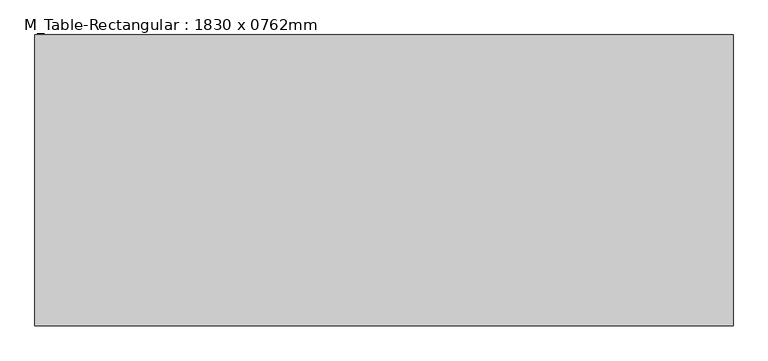
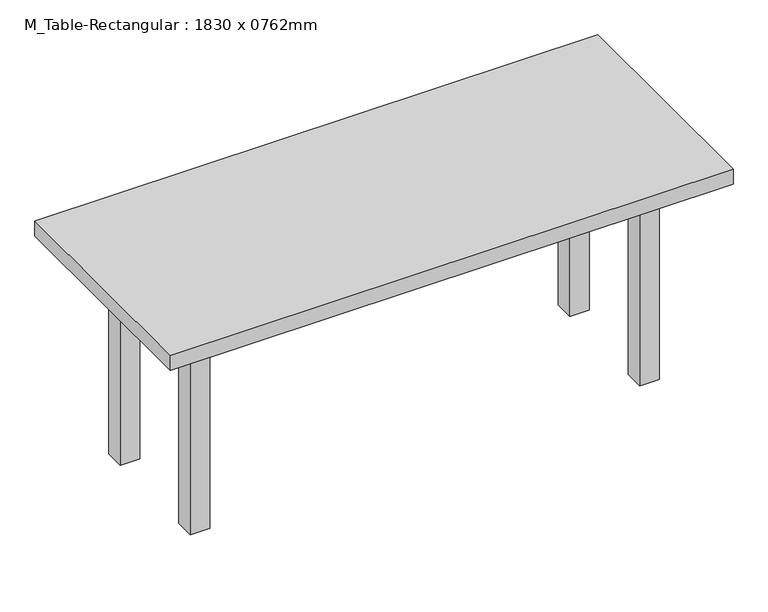
"""IFC4 building model written with IfcOpenShell, lengths in millimetres: furniture geometry, M_Table-Rectangular : 1830 x 0762mm."""

import ifcopenshell
import ifcopenshell.guid

model = None  # the IFC model being written
_history = None  # IfcOwnerHistory: only IFC2X3 demands one
_inside = {}  # id of a spatial element -> (the spatial element, [elements in it])
_under = {}  # id of a project, library or spatial element -> (it, [spatial elements below it])
_declared = {}  # id of a project -> (the project, [libraries it declares])
_typed = {}  # id of a type object -> (the type object, [elements of that type])
_made_of = {}  # id of a material, layer set ... -> (it, [elements and type objects made of it])


def new_model(schema):
    """Start an empty IFC model of exactly this schema.

    Asked for "IFC4X3", IfcOpenShell would pick the latest addendum, in which some entities
    have other attributes; the version numbers below select the first issue.
    IFC2X3 requires an IfcOwnerHistory on every rooted entity: one is made here for all.
    """
    global model, _history
    if schema == "IFC4X3":
        model = ifcopenshell.file(schema_version=(4, 3, 0, 0))
    else:
        model = ifcopenshell.file(schema=schema)
    _inside.clear()
    _under.clear()
    _declared.clear()
    _typed.clear()
    _made_of.clear()
    _history = None
    if model.schema == "IFC2X3":
        org = make("IfcOrganization", Name="unknown")
        user = make(
            "IfcPersonAndOrganization",
            ThePerson=make("IfcPerson", FamilyName="unknown"),
            TheOrganization=org,
        )
        app = make(
            "IfcApplication",
            ApplicationDeveloper=org,
            Version="unknown",
            ApplicationFullName="unknown",
            ApplicationIdentifier="unknown",
        )
        _history = make(
            "IfcOwnerHistory",
            OwningUser=user,
            OwningApplication=app,
            ChangeAction="ADDED",
            CreationDate=0,
        )
    return model


def make(cls, **values):
    """One entity of the class cls with the attributes given. An attribute that is None is left unset."""
    return model.create_entity(
        cls, **{name: value for name, value in values.items() if value is not None}
    )


def rooted(cls, **values):
    """An entity with a GlobalId (a new one), such as an element, a storey or a relation."""
    return make(cls, GlobalId=ifcopenshell.guid.new(), OwnerHistory=_history, **values)


def si_unit(unit_type, name, prefix=None):
    """IfcSIUnit, for example si_unit("LENGTHUNIT", "METRE", prefix="MILLI")."""
    return make("IfcSIUnit", UnitType=unit_type, Prefix=prefix, Name=name)


def assignment(units):
    """IfcUnitAssignment: the units of a project."""
    return None if units is None else make("IfcUnitAssignment", Units=units)


def point(xyz):
    """IfcCartesianPoint."""
    return None if xyz is None else make("IfcCartesianPoint", Coordinates=xyz)


def direction(xyz):
    """IfcDirection."""
    return None if xyz is None else make("IfcDirection", DirectionRatios=xyz)


def frame(location, z_axis=None, x_axis=None):
    """IfcAxis2Placement3D, a coordinate frame: its origin and axes. An axis left out is left unset."""
    return make(
        "IfcAxis2Placement3D",
        Location=point(location),
        Axis=direction(z_axis),
        RefDirection=direction(x_axis),
    )


def origin():
    """The frame at (0, 0, 0) with its axes left unset."""
    return frame((0.0, 0.0, 0.0))


def origin_with_axes():
    """The frame at (0, 0, 0) with the z axis (0, 0, 1) and the x axis (1, 0, 0) written out."""
    return frame((0.0, 0.0, 0.0), z_axis=(0.0, 0.0, 1.0), x_axis=(1.0, 0.0, 0.0))


def place(relative_to, where):
    """IfcLocalPlacement: puts the frame where relative to a parent placement (None: the world)."""
    return make(
        "IfcLocalPlacement", PlacementRelTo=relative_to, RelativePlacement=where
    )


def context(
    kind, dimensions, precision=None, world=None, true_north=None, identifier=None
):
    """IfcGeometricRepresentationContext, for example the 3D "Model" context."""
    return make(
        "IfcGeometricRepresentationContext",
        ContextIdentifier=identifier,
        ContextType=kind,
        CoordinateSpaceDimension=dimensions,
        Precision=precision,
        WorldCoordinateSystem=world,
        TrueNorth=true_north,
    )


def project(units=None, contexts=None):
    """IfcProject with its units and contexts."""
    return rooted(
        "IfcProject",
        Name="project",
        RepresentationContexts=contexts,
        UnitsInContext=assignment(units),
    )


def spatial(cls, under=None, at=None, **own):
    """A site, building, storey or space (cls), placed at a placement, below another one or the project."""
    s = rooted(cls, ObjectPlacement=at, **own)
    if under is not None:
        _under.setdefault(under.id(), (under, []))[1].append(s)
    return s


def polyline(points):
    """IfcPolyline through the points."""
    return make("IfcPolyline", Points=[point(p) for p in points])


def outline(outer, holes=None, kind="AREA"):
    """IfcArbitraryClosedProfileDef: a profile drawn as a closed curve; with holes, ...WithVoids."""
    if holes is None:
        return make("IfcArbitraryClosedProfileDef", ProfileType=kind, OuterCurve=outer)
    return make(
        "IfcArbitraryProfileDefWithVoids",
        ProfileType=kind,
        OuterCurve=outer,
        InnerCurves=holes,
    )


def extrude(swept, where, along, depth):
    """IfcExtrudedAreaSolid: the profile swept, set in the frame where, extruded along a direction by depth."""
    return make(
        "IfcExtrudedAreaSolid",
        SweptArea=swept,
        Position=where,
        ExtrudedDirection=direction(along),
        Depth=depth,
    )


def shape(context_of_items, identifier, shape_type, items):
    """IfcShapeRepresentation: the items that make up one representation, for example the "Body"."""
    return make(
        "IfcShapeRepresentation",
        ContextOfItems=context_of_items,
        RepresentationIdentifier=identifier,
        RepresentationType=shape_type,
        Items=items,
    )


def source(mapping_origin, context_of_items, identifier, shape_type, items):
    """IfcRepresentationMap: a shape defined once, which mapped items show again and again."""
    return make(
        "IfcRepresentationMap",
        MappingOrigin=mapping_origin,
        MappedRepresentation=shape(context_of_items, identifier, shape_type, items),
    )


def transform(
    local_origin,
    x_axis=None,
    y_axis=None,
    z_axis=None,
    scale=None,
    scale2=None,
    scale3=None,
    uniform=True,
):
    """IfcCartesianTransformationOperator3D, or its non-uniform kind. x_axis, y_axis, z_axis: its Axis1, 2, 3."""
    if uniform:
        return make(
            "IfcCartesianTransformationOperator3D",
            Axis1=direction(x_axis),
            Axis2=direction(y_axis),
            LocalOrigin=point(local_origin),
            Scale=scale,
            Axis3=direction(z_axis),
        )
    return make(
        "IfcCartesianTransformationOperator3DnonUniform",
        Axis1=direction(x_axis),
        Axis2=direction(y_axis),
        LocalOrigin=point(local_origin),
        Scale=scale,
        Axis3=direction(z_axis),
        Scale2=scale2,
        Scale3=scale3,
    )


def mapped(mapping_source, mapping_target):
    """IfcMappedItem: shows the shape of a source again, moved by a transform."""
    return make(
        "IfcMappedItem", MappingSource=mapping_source, MappingTarget=mapping_target
    )


def made_of(thing, what):
    """Note that an element or type object is made of a material, layer set ...; save() writes the relation."""
    if what is not None:
        _made_of.setdefault(what.id(), (what, []))[1].append(thing)
    return thing


def element(
    cls,
    number,
    at=None,
    inside=None,
    cuts=None,
    type_object=None,
    material=None,
    context=None,
    identifier="Body",
    shape_type=None,
    held_by="IfcProductDefinitionShape",
    body=None,
    shapes=None,
    **own,
):
    """One element of the class cls, such as IfcWall. Its Tag is "e" and its number.

    at: its placement. inside: the storey or other place that contains it. cuts: it is an
    opening in that element (IfcRelVoidsElement). A single representation is given by context,
    identifier, shape_type and body (its items); several are given by shapes. held_by: the class
    of the entity that holds the representations. save() writes the other relations.
    """
    e = rooted(cls, Tag="e%d" % number, ObjectPlacement=at, **own)
    if body is not None:
        shapes = [shape(context, identifier, shape_type, body)]
    if shapes is not None:
        e.Representation = make(held_by, Representations=shapes)
    if inside is not None:
        _inside.setdefault(inside.id(), (inside, []))[1].append(e)
    if cuts is not None:
        rooted(
            "IfcRelVoidsElement", RelatingBuildingElement=cuts, RelatedOpeningElement=e
        )
    if type_object is not None:
        _typed.setdefault(type_object.id(), (type_object, []))[1].append(e)
    return made_of(e, material)


def aggregate(whole, parts):
    """IfcRelAggregates: a whole, such as a stair, and the parts it consists of."""
    return rooted("IfcRelAggregates", RelatingObject=whole, RelatedObjects=parts)


def save(model, path):
    """Write the relations noted so far, then the file.

    IfcRelAggregates (storeys below a building ...), IfcRelContainedInSpatialStructure (elements
    in a storey), IfcRelDefinesByType, IfcRelAssociatesMaterial and IfcRelDeclares: one each for
    every whole, place, type object, material and project.
    """
    for whole, parts in _under.values():
        aggregate(whole, parts)
    for where, things in _inside.values():
        rooted(
            "IfcRelContainedInSpatialStructure",
            RelatedElements=things,
            RelatingStructure=where,
        )
    for kind, things in _typed.values():
        rooted("IfcRelDefinesByType", RelatedObjects=things, RelatingType=kind)
    for what, things in _made_of.values():
        rooted("IfcRelAssociatesMaterial", RelatedObjects=things, RelatingMaterial=what)
    for by, libraries in _declared.values():
        rooted("IfcRelDeclares", RelatingContext=by, RelatedDefinitions=libraries)
    model.write(path)


def m_table_rectangular_1830_x_0762mm_ec068ed4(model_context):
    return source(origin(), model_context, "Body", "SweptSolid", [
        extrude(outline(polyline([(699.1, -190.5), (-699.1, -190.5), (-699.1, -165.1), (699.1, -165.1), (699.1, -190.5)])), frame((0.0, 0.0, 609.6), z_axis=(0.0, 0.0, 1.0), x_axis=(1.0, 0.0, 0.0)), (0.0, 0.0, 1.0), 101.6),
        extrude(outline(polyline([(699.1, 190.5), (699.1, 165.1), (-699.1, 165.1), (-699.1, 190.5), (699.1, 190.5)])), frame((0.0, 0.0, 609.6), z_axis=(0.0, 0.0, 1.0), x_axis=(1.0, 0.0, 0.0)), (0.0, 0.0, 1.0), 101.6),
        extrude(outline(polyline([(-711.8, 165.1), (-711.8, -165.1), (-737.2, -165.1), (-737.2, 165.1), (-711.8, 165.1)])), frame((0.0, 0.0, 609.6), z_axis=(0.0, 0.0, 1.0), x_axis=(1.0, 0.0, 0.0)), (0.0, 0.0, 1.0), 101.6),
        extrude(outline(polyline([(711.8, 165.1), (737.2, 165.1), (737.2, -165.1), (711.8, -165.1), (711.8, 165.1)])), frame((0.0, 0.0, 609.6), z_axis=(0.0, 0.0, 1.0), x_axis=(1.0, 0.0, 0.0)), (0.0, 0.0, 1.0), 101.6),
        extrude(outline(polyline([(915.0, -381.0), (-915.0, -381.0), (-915.0, 381.0), (915.0, 381.0), (915.0, -381.0)])), frame((0.0, 0.0, 711.2), z_axis=(0.0, 0.0, 1.0), x_axis=(1.0, 0.0, 0.0)), (0.0, 0.0, 1.0), 50.8),
        extrude(outline(polyline([(-699.1, -228.6), (-762.6, -228.6), (-762.6, -165.1), (-699.1, -165.1), (-699.1, -228.6)])), origin_with_axes(), (0.0, 0.0, 1.0), 711.2),
        extrude(outline(polyline([(699.1, -228.6), (699.1, -165.1), (762.6, -165.1), (762.6, -228.6), (699.1, -228.6)])), origin_with_axes(), (0.0, 0.0, 1.0), 711.2),
        extrude(outline(polyline([(-699.1, 228.6), (-699.1, 165.1), (-762.6, 165.1), (-762.6, 228.6), (-699.1, 228.6)])), origin_with_axes(), (0.0, 0.0, 1.0), 711.2),
        extrude(outline(polyline([(699.1, 228.6), (762.6, 228.6), (762.6, 165.1), (699.1, 165.1), (699.1, 228.6)])), origin_with_axes(), (0.0, 0.0, 1.0), 711.2),
    ])


if __name__ == "__main__":
    model = new_model("IFC4")
    model_context = context("Model", 3, world=origin())
    ifc_project = project(units=[si_unit("LENGTHUNIT", "METRE", prefix="MILLI")], contexts=[model_context])
    site = spatial("IfcSite", under=ifc_project)
    building = spatial("IfcBuilding", under=site)
    placement = place(None, origin())
    m_table_rectangular_1830_x_0762mm_shape = m_table_rectangular_1830_x_0762mm_ec068ed4(model_context)
    element("IfcFurniture", 1, ObjectType="M_Table-Rectangular : 1830 x 0762mm", at=placement, inside=building, context=model_context, shape_type="MappedRepresentation", body=[
        mapped(m_table_rectangular_1830_x_0762mm_shape, transform((0.0, 0.0, 0.0), x_axis=(1.0, 0.0, 0.0), y_axis=(0.0, 1.0, 0.0), z_axis=(0.0, 0.0, 1.0))),
    ])
    save(model, "model.ifc")

# Revit data of these elements
# Type "M_Table-Rectangular : 1830 x 0762mm"
#   Height = 762 mm
#   Length = 1830 mm
#   Width = 762 mm
#   Base Material = Birch
#   Top Material = Birch
#   Default Elevation = 0
# Element 1 (IfcFurniture, "M_Table-Rectangular : 1830 x 0762mm")
#   Materials on its faces: "Birch"
# Materials
#   "Birch": class "Wood", colour RGB 224 178 126, transparency 0, Description = "Betula Alleghaniensis", Cost = 0
